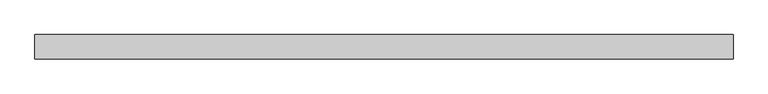
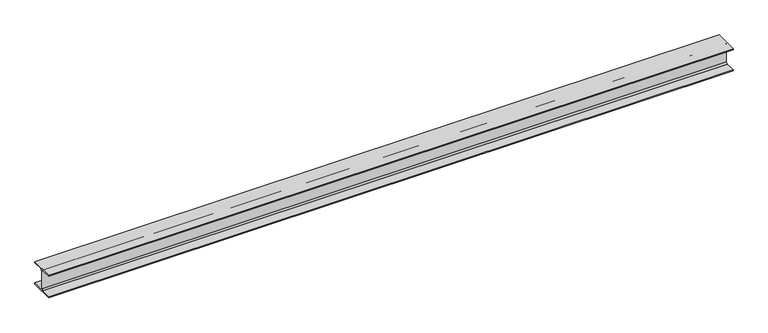
"""IFC4 building model written with IfcOpenShell, lengths in millimetres: beam geometry, 0912_Steel Framing_H-KSD3502 : H_SB_ASB_H-300x300x10x15."""

from ifc_helpers import new_model, si_unit, point, frame, frame_2d, origin, place, context, project, spatial, polyline, circle_curve, trimmed, segment, composite_curve, outline, extrude, source, transform, mapped, element, save


def beam_276f2b7d(model_context):
    return source(origin(), model_context, "Body", "SweptSolid", [
        extrude(outline(composite_curve([segment(polyline([(150.0, -135.0), (150.0, -150.0), (-150.0, -150.0), (-150.0, -135.0), (-23.0, -135.0)]), True, "CONTINUOUS"), segment(trimmed(circle_curve(frame_2d((-23.0, -117.0)), 18.0), [point((-23.0, -135.0))], [point((-5.0, -117.0))], True, "CARTESIAN"), True, "CONTINUOUS"), segment(polyline([(-5.0, -117.0), (-5.0, 117.0)]), True, "CONTINUOUS"), segment(trimmed(circle_curve(frame_2d((-23.0, 117.0)), 18.0), [point((-5.0, 117.0))], [point((-23.0, 135.0))], True, "CARTESIAN"), True, "CONTINUOUS"), segment(polyline([(-23.0, 135.0), (-150.0, 135.0), (-150.0, 150.0), (150.0, 150.0), (150.0, 135.0), (23.0, 135.0)]), True, "CONTINUOUS"), segment(trimmed(circle_curve(frame_2d((23.0, 117.0)), 18.0), [point((23.0, 135.0))], [point((5.0, 117.0))], True, "CARTESIAN"), True, "CONTINUOUS"), segment(polyline([(5.0, 117.0), (5.0, -117.0)]), True, "CONTINUOUS"), segment(trimmed(circle_curve(frame_2d((23.0, -117.0)), 18.0), [point((5.0, -117.0))], [point((23.0, -135.0))], True, "CARTESIAN"), True, "CONTINUOUS"), segment(polyline([(23.0, -135.0), (150.0, -135.0)]), True, "CONTINUOUS")], self_intersect=False)), frame((-4272.9251782, 0.0, 0.0), z_axis=(1.0, 0.0, 0.0), x_axis=(0.0, 1.0, 0.0)), (0.0, 0.0, 1.0), 8647.1704515),
    ])


if __name__ == "__main__":
    model = new_model("IFC4")
    model_context = context("Model", 3, world=origin())
    ifc_project = project(units=[si_unit("LENGTHUNIT", "METRE", prefix="MILLI")], contexts=[model_context])
    site = spatial("IfcSite", under=ifc_project)
    building = spatial("IfcBuilding", under=site)
    placement = place(None, origin())
    beam_shape = beam_276f2b7d(model_context)
    element("IfcBeam", 1, ObjectType="0912_Steel Framing_H-KSD3502 : H_SB_ASB_H-300x300x10x15", at=placement, inside=building, context=model_context, shape_type="MappedRepresentation", body=[
        mapped(beam_shape, transform((0.0, 0.0, 0.0), x_axis=(1.0, 0.0, 0.0), y_axis=(0.0, 1.0, 0.0), z_axis=(0.0, 0.0, 1.0))),
    ])
    save(model, "model.ifc")

# Revit data of these elements
# Type "0912_Steel Framing_H-KSD3502 : H_SB_ASB_H-300x300x10x15"
#   H_WM Code_1 = "S01AA001-00001 | Main Steel Structure Fabrication Work | Shelter/Building | Heavy Steel - Standard (Weight≥90KG/M) | Material: (   )"
#   H_WM Code_2 = "S03AA027-00001 | Main Steel Structure Erection Work | Shelter/Building | Heavy Steel (Weight≥90KG/M) | Material: (   )"
#   H_WM Code_3 = "S01AA010-00001 | Main Steel Structure Fabrication Work | Shelter/Building | Steel Painting/Coating | for Non-Fireproofed Steel Surface, Surface Preparation, Primer, Second & Final Coat | Material: (   )"
#   H_Q'ty Cal Type Tag = "SB-Q2"
#   Width = 30.0 cm
#   Web Thickness = 1.0 cm
#   Web Fillet = 1.8 cm
#   Warping Constant = 1370000.0 cm⁶
#   W = 0
#   Torsional Moment of Inertia = 77.00 cm⁴
#   Section Area = 119.8 cm²
#   Plastic Modulus weak axis = 684.0 cm³
#   Plastic Modulus strong axis = 1500.0 cm³
#   Perimeter = 1.75 m²/m
#   Nominal Weight = 94.00 kgf/m
#   Moment of Inertia weak axis = 6750.00 cm⁴
#   Moment of Inertia strong axis = 20400.00 cm⁴
#   Height = 30.0 cm
#   Flange Thickness = 1.5 cm
#   Elastic Modulus weak axis = 450.0 cm³
#   Elastic Modulus strong axis = 1360.0 cm³
#   Centroid Vertical = 15.0 cm
#   Centroid Horizontal = 15.0 cm
#   Ix = 204000000
#   Length [instance default] = 1.5240 m
#   Zx = 1500000
#   b = 0.3000 m
#   h = 0.3000 m
#   r = 0.0180 m
#   s = 0.0100 m
#   t = 0.0150 m
#   A = 0.01198 m²
#   Structural Material [instance default] = Steel, 45-345
#   Assembly Code = ""
# Element 1 (IfcBeam, "0912_Steel Framing_H-KSD3502 : H_SB_ASB_H-300x300x10x15")
#   Structural Material = none
# Materials
#   "Steel, 45-345": class "Metal", colour RGB 189 187 185, transparency 0, Description = "Steel 345 MPa", Cost = 0
